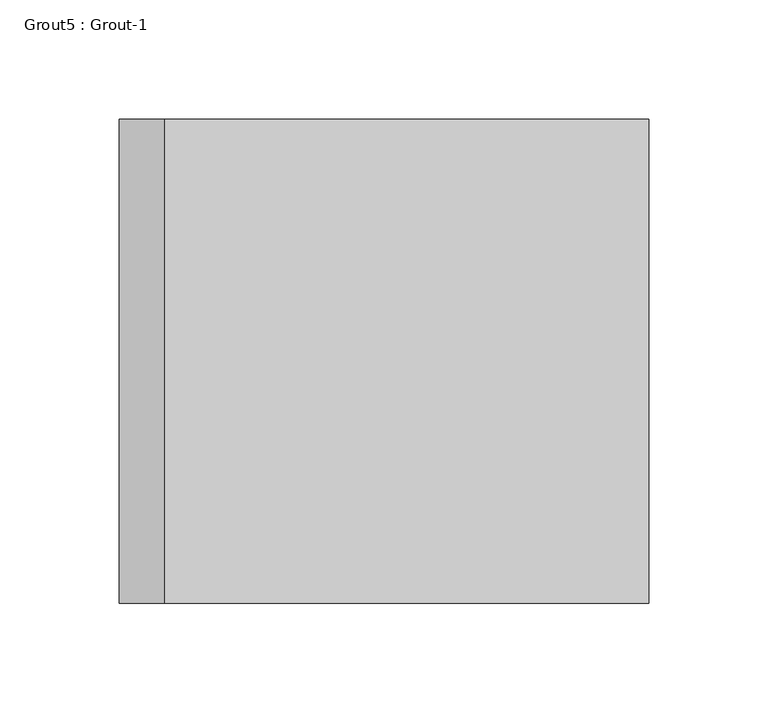
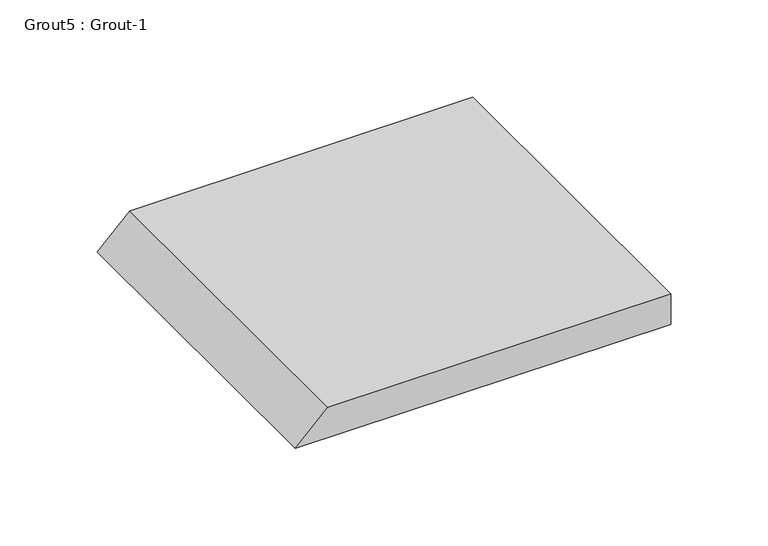
"""IFC4 building model written with IfcOpenShell, lengths in millimetres: proxy geometry, Grout5 : Grout-1."""

from ifc_helpers import new_model, si_unit, frame, origin, place, context, project, spatial, polyline, outline, extrude, source, transform, mapped, element, save


def grout5_grout_1_e9fd96e3(model_context):
    return source(origin(), model_context, "Body", "SweptSolid", [
        extrude(outline(polyline([(19.05, 590115.4434739), (0.0, 590096.3934739), (0.0, 590318.6434739), (19.05, 590318.6434739), (19.05, 590115.4434739)])), frame((0.0, -534144.2913841, 0.0), z_axis=(0.0, 1.0, 0.0), x_axis=(0.0, 0.0, 1.0)), (0.0, 0.0, 1.0), 203.2),
    ])


if __name__ == "__main__":
    model = new_model("IFC4")
    model_context = context("Model", 3, world=origin())
    ifc_project = project(units=[si_unit("LENGTHUNIT", "METRE", prefix="MILLI")], contexts=[model_context])
    site = spatial("IfcSite", under=ifc_project)
    building = spatial("IfcBuilding", under=site)
    placement = place(None, origin())
    grout5_grout_1_shape = grout5_grout_1_e9fd96e3(model_context)
    element("IfcBuildingElementProxy", 1, Name="Grout5 : Grout-1", ObjectType="Grout5 : Grout-1", at=placement, inside=building, context=model_context, shape_type="MappedRepresentation", body=[
        mapped(grout5_grout_1_shape, transform((0.0, 0.0, 0.0), x_axis=(1.0, 0.0, 0.0), y_axis=(0.0, 1.0, 0.0), z_axis=(0.0, 0.0, 1.0))),
    ])
    save(model, "model.ifc")

# Revit data of these elements
# Element 1 (IfcBuildingElementProxy, "Grout5 : Grout-1")
#   Materials on its faces: "3/4\" NON SHRINK GROUT"
# Materials
#   "3/4\" NON SHRINK GROUT": class "Generic", colour RGB 145 145 143, transparency 0, Cost = 0
